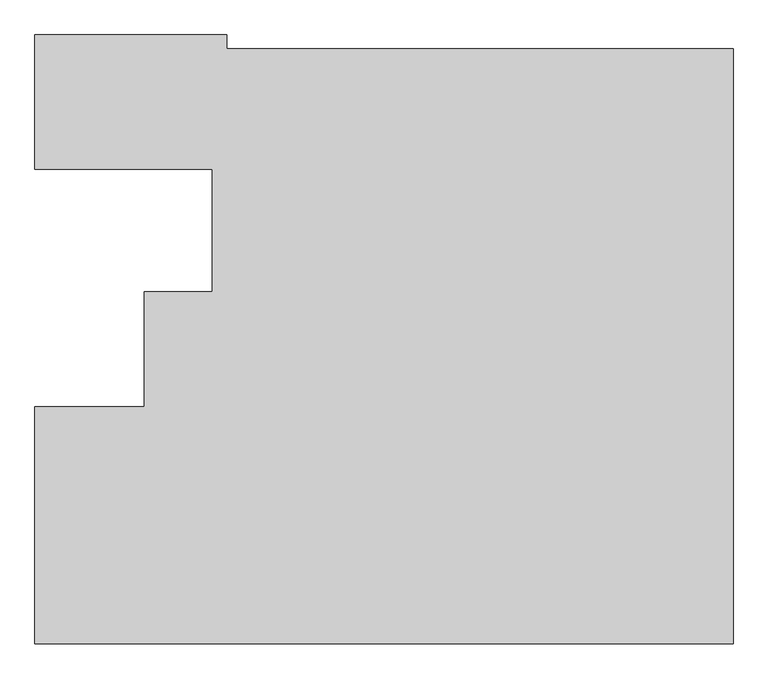
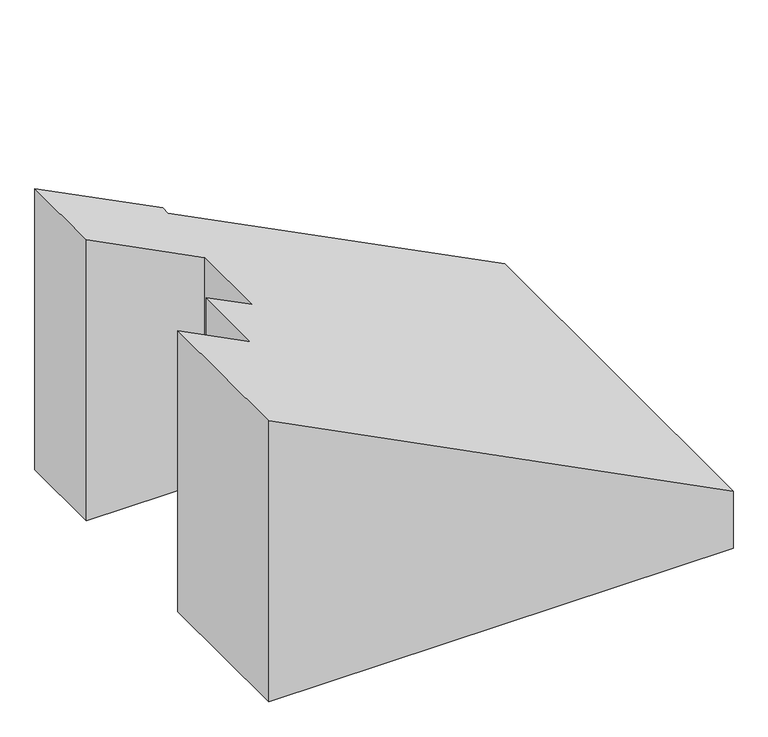
"""IFC4 building model written with IfcOpenShell, lengths in millimetres: proxy geometry, 0_3d_modell."""

from ifc_helpers import new_model, si_unit, origin, place, context, project, spatial, faceted_brep, source, transform, mapped, element, save


def generic_models_e99fb198(model_context):
    return source(origin(), model_context, "Body", "Brep", [
        faceted_brep([(1800.0, 5582.8619019, 3273.5797924), (1800.0, 5712.8619019, 3273.5797924), (0.0, 5712.8619019, 4190.7256015), (0.0, 4452.8619019, 4190.7256015), (1665.0, 4452.8619019, 3342.3657281), (1665.0, 3302.8619019, 3342.3657281), (1025.0, 3302.8619019, 3668.4620158), (1025.0, 2223.2600653, 3668.4620158), (0.0, 2223.2600653, 4190.7256015), (0.0, 0.0, 4190.7256015), (6550.0, 0.0, 853.3339073), (6550.0, 5582.8619019, 853.3339073), (1025.0, 3302.8619019, 0.0), (1025.0, 2223.2600653, 0.0), (1665.0, 3302.8619019, 0.0), (1665.0, 4452.8619019, 0.0), (0.0, 4452.8619019, 0.0), (1800.0, 5712.8619019, 0.0), (0.0, 5712.8619019, 0.0), (1800.0, 5582.8619019, 0.0), (6550.0, 5582.8619019, 0.0), (6550.0, 0.0, 0.0), (0.0, 0.0, 0.0), (0.0, 2223.2600653, 0.0)], [[[0, 1, 2, 3, 4, 5, 6, 7, 8, 9, 10, 11]], [[7, 6, 12, 13]], [[6, 5, 14, 12]], [[5, 4, 15, 14]], [[4, 3, 16, 15]], [[2, 1, 17, 18]], [[1, 0, 19, 17]], [[0, 11, 20, 19]], [[11, 10, 21, 20]], [[10, 9, 22, 21]], [[23, 22, 9, 8]], [[8, 7, 13, 23]], [[18, 16, 3, 2]], [[18, 17, 19, 20, 21, 22, 23, 13, 12, 14, 15, 16]]]),
    ])


if __name__ == "__main__":
    model = new_model("IFC4")
    model_context = context("Model", 3, world=origin())
    ifc_project = project(units=[si_unit("LENGTHUNIT", "METRE", prefix="MILLI")], contexts=[model_context])
    site = spatial("IfcSite", under=ifc_project)
    building = spatial("IfcBuilding", under=site)
    placement = place(None, origin())
    generic_models_shape = generic_models_e99fb198(model_context)
    element("IfcBuildingElementProxy", 1, Name="0_3d_modell", ObjectType="0_3d_modell", at=placement, inside=building, context=model_context, shape_type="MappedRepresentation", body=[
        mapped(generic_models_shape, transform((0.0, 0.0, 0.0), x_axis=(1.0, 0.0, 0.0), y_axis=(0.0, 1.0, 0.0), z_axis=(0.0, 0.0, 1.0))),
    ])
    save(model, "model.ifc")

# Revit data of these elements
# Element 1 (IfcBuildingElementProxy, "0_3d_modell")
#   Materials on its faces: "*1"
# Materials
#   "*1": class "Unassigned", colour RGB 175 175 175, transparency 0
